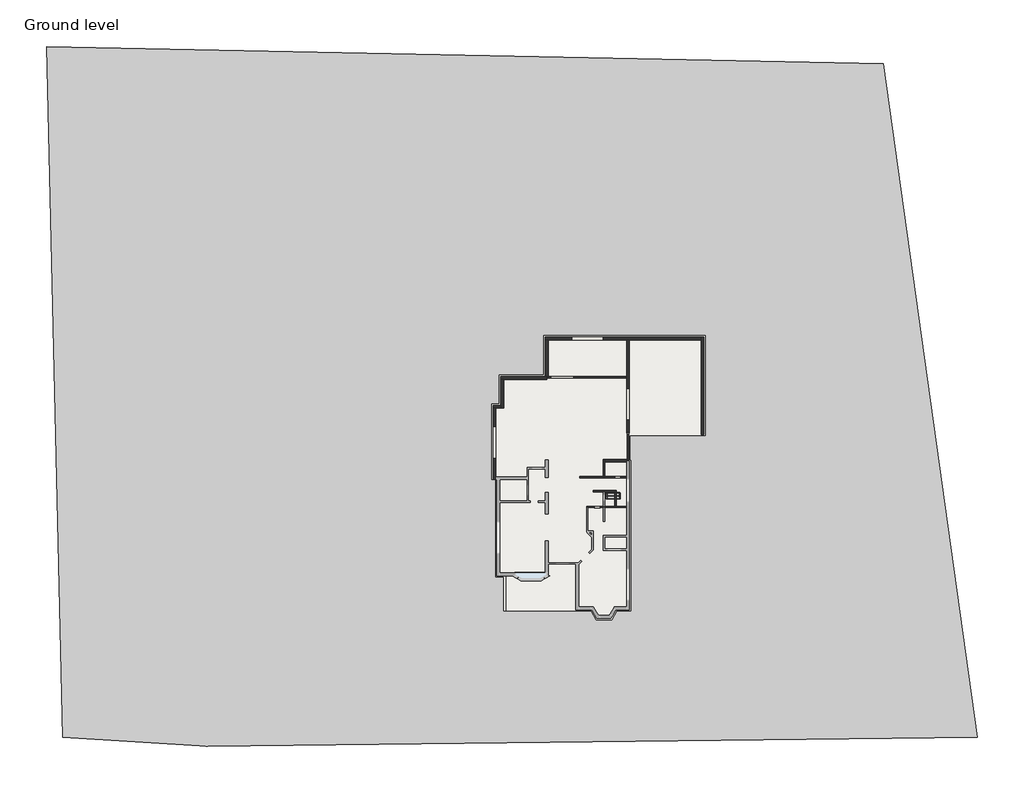
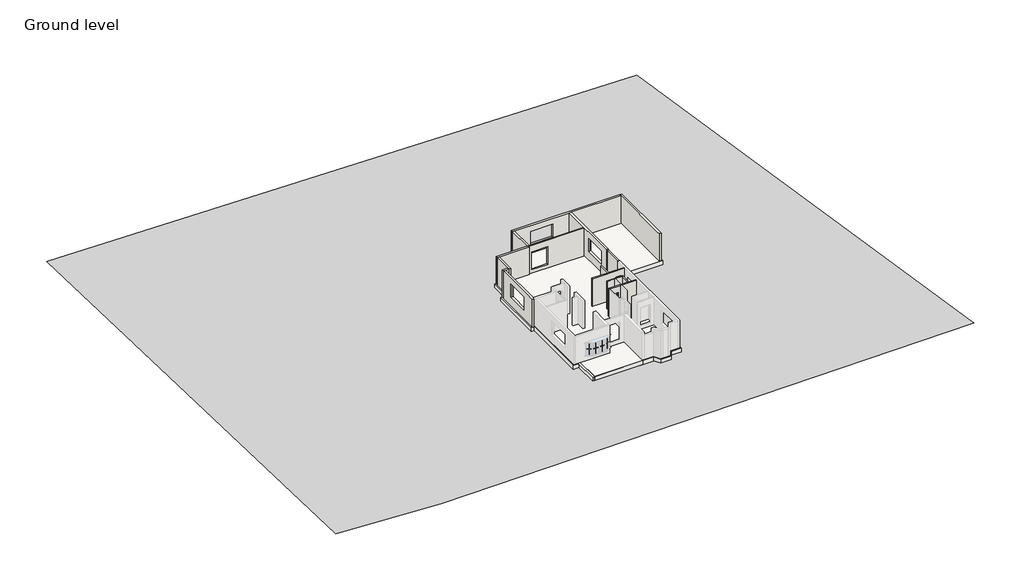
# One storey, part 2 of 2: 16 walls, 6 proxies, 2 members, 2 railings, 2 slabs, 1 stair flight.
"""IFC4 building model written with IfcOpenShell, lengths in millimetres."""

import ifcopenshell
import ifcopenshell.guid

model = None  # the IFC model being written
_history = None  # IfcOwnerHistory: only IFC2X3 demands one
_inside = {}  # id of a spatial element -> (the spatial element, [elements in it])
_under = {}  # id of a project, library or spatial element -> (it, [spatial elements below it])
_declared = {}  # id of a project -> (the project, [libraries it declares])
_typed = {}  # id of a type object -> (the type object, [elements of that type])
_made_of = {}  # id of a material, layer set ... -> (it, [elements and type objects made of it])


def new_model(schema):
    """Start an empty IFC model of exactly this schema.

    Asked for "IFC4X3", IfcOpenShell would pick the latest addendum, in which some entities
    have other attributes; the version numbers below select the first issue.
    IFC2X3 requires an IfcOwnerHistory on every rooted entity: one is made here for all.
    """
    global model, _history
    if schema == "IFC4X3":
        model = ifcopenshell.file(schema_version=(4, 3, 0, 0))
    else:
        model = ifcopenshell.file(schema=schema)
    _inside.clear()
    _under.clear()
    _declared.clear()
    _typed.clear()
    _made_of.clear()
    _history = None
    if model.schema == "IFC2X3":
        org = make("IfcOrganization", Name="unknown")
        user = make(
            "IfcPersonAndOrganization",
            ThePerson=make("IfcPerson", FamilyName="unknown"),
            TheOrganization=org,
        )
        app = make(
            "IfcApplication",
            ApplicationDeveloper=org,
            Version="unknown",
            ApplicationFullName="unknown",
            ApplicationIdentifier="unknown",
        )
        _history = make(
            "IfcOwnerHistory",
            OwningUser=user,
            OwningApplication=app,
            ChangeAction="ADDED",
            CreationDate=0,
        )
    return model


def make(cls, **values):
    """One entity of the class cls with the attributes given. An attribute that is None is left unset."""
    return model.create_entity(
        cls, **{name: value for name, value in values.items() if value is not None}
    )


def rooted(cls, **values):
    """An entity with a GlobalId (a new one), such as an element, a storey or a relation."""
    return make(cls, GlobalId=ifcopenshell.guid.new(), OwnerHistory=_history, **values)


def si_unit(unit_type, name, prefix=None):
    """IfcSIUnit, for example si_unit("LENGTHUNIT", "METRE", prefix="MILLI")."""
    return make("IfcSIUnit", UnitType=unit_type, Prefix=prefix, Name=name)


def assignment(units):
    """IfcUnitAssignment: the units of a project."""
    return None if units is None else make("IfcUnitAssignment", Units=units)


def point(xyz):
    """IfcCartesianPoint."""
    return None if xyz is None else make("IfcCartesianPoint", Coordinates=xyz)


def direction(xyz):
    """IfcDirection."""
    return None if xyz is None else make("IfcDirection", DirectionRatios=xyz)


def frame(location, z_axis=None, x_axis=None):
    """IfcAxis2Placement3D, a coordinate frame: its origin and axes. An axis left out is left unset."""
    return make(
        "IfcAxis2Placement3D",
        Location=point(location),
        Axis=direction(z_axis),
        RefDirection=direction(x_axis),
    )


def frame_2d(location, x_axis=None):
    """IfcAxis2Placement2D, a coordinate frame in the plane: its origin and x axis."""
    return make(
        "IfcAxis2Placement2D", Location=point(location), RefDirection=direction(x_axis)
    )


def origin():
    """The frame at (0, 0, 0) with its axes left unset."""
    return frame((0.0, 0.0, 0.0))


def origin_with_axes():
    """The frame at (0, 0, 0) with the z axis (0, 0, 1) and the x axis (1, 0, 0) written out."""
    return frame((0.0, 0.0, 0.0), z_axis=(0.0, 0.0, 1.0), x_axis=(1.0, 0.0, 0.0))


def place(relative_to, where):
    """IfcLocalPlacement: puts the frame where relative to a parent placement (None: the world)."""
    return make(
        "IfcLocalPlacement", PlacementRelTo=relative_to, RelativePlacement=where
    )


def context(
    kind, dimensions, precision=None, world=None, true_north=None, identifier=None
):
    """IfcGeometricRepresentationContext, for example the 3D "Model" context."""
    return make(
        "IfcGeometricRepresentationContext",
        ContextIdentifier=identifier,
        ContextType=kind,
        CoordinateSpaceDimension=dimensions,
        Precision=precision,
        WorldCoordinateSystem=world,
        TrueNorth=true_north,
    )


def project(units=None, contexts=None):
    """IfcProject with its units and contexts."""
    return rooted(
        "IfcProject",
        Name="project",
        RepresentationContexts=contexts,
        UnitsInContext=assignment(units),
    )


def spatial(cls, under=None, at=None, **own):
    """A site, building, storey or space (cls), placed at a placement, below another one or the project."""
    s = rooted(cls, ObjectPlacement=at, **own)
    if under is not None:
        _under.setdefault(under.id(), (under, []))[1].append(s)
    return s


def polyline(points):
    """IfcPolyline through the points."""
    return make("IfcPolyline", Points=[point(p) for p in points])


def point_list(points):
    """IfcCartesianPointList2D or 3D."""
    cls = (
        "IfcCartesianPointList2D" if len(points[0]) == 2 else "IfcCartesianPointList3D"
    )
    return make(cls, CoordList=points)


def circle_curve(where, radius):
    """IfcCircle in the frame where."""
    return make("IfcCircle", Position=where, Radius=radius)


def trimmed(basis, trim1, trim2, sense, master):
    """IfcTrimmedCurve: the piece of a basis curve between two trims."""
    return make(
        "IfcTrimmedCurve",
        BasisCurve=basis,
        Trim1=trim1,
        Trim2=trim2,
        SenseAgreement=sense,
        MasterRepresentation=master,
    )


def segment(curve, same_sense, transition):
    """IfcCompositeCurveSegment."""
    return make(
        "IfcCompositeCurveSegment",
        Transition=transition,
        SameSense=same_sense,
        ParentCurve=curve,
    )


def composite_curve(segments, self_intersect=None):
    """IfcCompositeCurve: segments joined end to end."""
    return make("IfcCompositeCurve", Segments=segments, SelfIntersect=self_intersect)


def outline(outer, holes=None, kind="AREA"):
    """IfcArbitraryClosedProfileDef: a profile drawn as a closed curve; with holes, ...WithVoids."""
    if holes is None:
        return make("IfcArbitraryClosedProfileDef", ProfileType=kind, OuterCurve=outer)
    return make(
        "IfcArbitraryProfileDefWithVoids",
        ProfileType=kind,
        OuterCurve=outer,
        InnerCurves=holes,
    )


def extrude(swept, where, along, depth):
    """IfcExtrudedAreaSolid: the profile swept, set in the frame where, extruded along a direction by depth."""
    return make(
        "IfcExtrudedAreaSolid",
        SweptArea=swept,
        Position=where,
        ExtrudedDirection=direction(along),
        Depth=depth,
    )


def faces_of(points, faces, orient=None, outer=None):
    """IfcFace entities. A face is a list of loops; a loop is a list of indices into points, from 0.

    orient and outer hold one flag for each loop. By default every Orientation is true, the
    first loop of a face is its IfcFaceOuterBound and the others are IfcFaceBound.
    """
    made = []
    for i, loops in enumerate(faces):
        bounds = []
        for j, loop in enumerate(loops):
            is_outer = j == 0 if outer is None else outer[i][j]
            bounds.append(
                make(
                    "IfcFaceOuterBound" if is_outer else "IfcFaceBound",
                    Bound=make("IfcPolyLoop", Polygon=[points[k] for k in loop]),
                    Orientation=True if orient is None else orient[i][j],
                )
            )
        made.append(make("IfcFace", Bounds=bounds))
    return made


def faceted_brep(points, faces, orient=None, outer=None, voids=None):
    """IfcFacetedBrep: a solid bounded by flat faces; with voids (closed shells), ...WithVoids."""
    shared = [point(p) for p in points]
    hull = make("IfcClosedShell", CfsFaces=faces_of(shared, faces, orient, outer))
    if voids is None:
        return make("IfcFacetedBrep", Outer=hull)
    return make(
        "IfcFacetedBrepWithVoids",
        Outer=hull,
        Voids=[
            make(cls, CfsFaces=faces_of(shared, fs, o, b)) for cls, fs, o, b in voids
        ],
    )


def triangles(points, corners, closed=None, point_numbers=None):
    """IfcTriangulatedFaceSet: each triangle names its three corners, points numbered from 1."""
    return make(
        "IfcTriangulatedFaceSet",
        Coordinates=point_list(points),
        Closed=closed,
        CoordIndex=corners,
        PnIndex=point_numbers,
    )


def shape(context_of_items, identifier, shape_type, items):
    """IfcShapeRepresentation: the items that make up one representation, for example the "Body"."""
    return make(
        "IfcShapeRepresentation",
        ContextOfItems=context_of_items,
        RepresentationIdentifier=identifier,
        RepresentationType=shape_type,
        Items=items,
    )


def source(mapping_origin, context_of_items, identifier, shape_type, items):
    """IfcRepresentationMap: a shape defined once, which mapped items show again and again."""
    return make(
        "IfcRepresentationMap",
        MappingOrigin=mapping_origin,
        MappedRepresentation=shape(context_of_items, identifier, shape_type, items),
    )


def transform(
    local_origin,
    x_axis=None,
    y_axis=None,
    z_axis=None,
    scale=None,
    scale2=None,
    scale3=None,
    uniform=True,
):
    """IfcCartesianTransformationOperator3D, or its non-uniform kind. x_axis, y_axis, z_axis: its Axis1, 2, 3."""
    if uniform:
        return make(
            "IfcCartesianTransformationOperator3D",
            Axis1=direction(x_axis),
            Axis2=direction(y_axis),
            LocalOrigin=point(local_origin),
            Scale=scale,
            Axis3=direction(z_axis),
        )
    return make(
        "IfcCartesianTransformationOperator3DnonUniform",
        Axis1=direction(x_axis),
        Axis2=direction(y_axis),
        LocalOrigin=point(local_origin),
        Scale=scale,
        Axis3=direction(z_axis),
        Scale2=scale2,
        Scale3=scale3,
    )


def mapped(mapping_source, mapping_target):
    """IfcMappedItem: shows the shape of a source again, moved by a transform."""
    return make(
        "IfcMappedItem", MappingSource=mapping_source, MappingTarget=mapping_target
    )


def made_of(thing, what):
    """Note that an element or type object is made of a material, layer set ...; save() writes the relation."""
    if what is not None:
        _made_of.setdefault(what.id(), (what, []))[1].append(thing)
    return thing


def element(
    cls,
    number,
    at=None,
    inside=None,
    cuts=None,
    type_object=None,
    material=None,
    context=None,
    identifier="Body",
    shape_type=None,
    held_by="IfcProductDefinitionShape",
    body=None,
    shapes=None,
    **own,
):
    """One element of the class cls, such as IfcWall. Its Tag is "e" and its number.

    at: its placement. inside: the storey or other place that contains it. cuts: it is an
    opening in that element (IfcRelVoidsElement). A single representation is given by context,
    identifier, shape_type and body (its items); several are given by shapes. held_by: the class
    of the entity that holds the representations. save() writes the other relations.
    """
    e = rooted(cls, Tag="e%d" % number, ObjectPlacement=at, **own)
    if body is not None:
        shapes = [shape(context, identifier, shape_type, body)]
    if shapes is not None:
        e.Representation = make(held_by, Representations=shapes)
    if inside is not None:
        _inside.setdefault(inside.id(), (inside, []))[1].append(e)
    if cuts is not None:
        rooted(
            "IfcRelVoidsElement", RelatingBuildingElement=cuts, RelatedOpeningElement=e
        )
    if type_object is not None:
        _typed.setdefault(type_object.id(), (type_object, []))[1].append(e)
    return made_of(e, material)


def aggregate(whole, parts):
    """IfcRelAggregates: a whole, such as a stair, and the parts it consists of."""
    return rooted("IfcRelAggregates", RelatingObject=whole, RelatedObjects=parts)


def save(model, path):
    """Write the relations noted so far, then the file.

    IfcRelAggregates (storeys below a building ...), IfcRelContainedInSpatialStructure (elements
    in a storey), IfcRelDefinesByType, IfcRelAssociatesMaterial and IfcRelDeclares: one each for
    every whole, place, type object, material and project.
    """
    for whole, parts in _under.values():
        aggregate(whole, parts)
    for where, things in _inside.values():
        rooted(
            "IfcRelContainedInSpatialStructure",
            RelatedElements=things,
            RelatingStructure=where,
        )
    for kind, things in _typed.values():
        rooted("IfcRelDefinesByType", RelatedObjects=things, RelatingType=kind)
    for what, things in _made_of.values():
        rooted("IfcRelAssociatesMaterial", RelatedObjects=things, RelatingMaterial=what)
    for by, libraries in _declared.values():
        rooted("IfcRelDeclares", RelatingContext=by, RelatedDefinitions=libraries)
    model.write(path)


def m_muntin_pattern_2x2_m_muntin_pattern_2x2_0b9f2fee(model_context):
    return source(origin(), model_context, "Body", "SweptSolid", [
        extrude(outline(polyline([(686.5, -6.35), (686.5, -246.1999152), (673.8, -246.1999152), (673.8, -6.35), (0.0, -6.35), (0.0, 6.35), (673.8, 6.35), (673.8, 246.1999152), (686.5, 246.1999152), (686.5, 6.35), (1360.3, 6.35), (1360.3, -6.35), (686.5, -6.35)])), frame((0.0, 9.525, 0.0), z_axis=(0.0, 1.0, 0.0), x_axis=(0.0, 0.0, 1.0)), (0.0, 0.0, 1.0), 12.7),
        extrude(outline(polyline([(686.5, -6.35), (686.5, -246.1999152), (673.8, -246.1999152), (673.8, -6.35), (0.0, -6.35), (0.0, 6.35), (673.8, 6.35), (673.8, 246.1999152), (686.5, 246.1999152), (686.5, 6.35), (1360.3, 6.35), (1360.3, -6.35), (686.5, -6.35)])), frame((0.0, -22.225, 0.0), z_axis=(0.0, 1.0, 0.0), x_axis=(0.0, 0.0, 1.0)), (0.0, 0.0, 1.0), 12.7),
    ])


def m_muntin_pattern_2x2_m_muntin_pattern_2x2_98e5798c(model_context):
    return source(origin(), model_context, "Body", "SweptSolid", [
        extrude(outline(polyline([(686.5, -6.35), (686.5, -223.0), (673.8, -223.0), (673.8, -6.35), (0.0, -6.35), (0.0, 6.35), (673.8, 6.35), (673.8, 223.0), (686.5, 223.0), (686.5, 6.35), (1360.3, 6.35), (1360.3, -6.35), (686.5, -6.35)])), frame((0.0, 9.525, 0.0), z_axis=(0.0, 1.0, 0.0), x_axis=(0.0, 0.0, 1.0)), (0.0, 0.0, 1.0), 12.7),
        extrude(outline(polyline([(686.5, -6.35), (686.5, -223.0), (673.8, -223.0), (673.8, -6.35), (0.0, -6.35), (0.0, 6.35), (673.8, 6.35), (673.8, 223.0), (686.5, 223.0), (686.5, 6.35), (1360.3, 6.35), (1360.3, -6.35), (686.5, -6.35)])), frame((0.0, -22.225, 0.0), z_axis=(0.0, 1.0, 0.0), x_axis=(0.0, 0.0, 1.0)), (0.0, 0.0, 1.0), 12.7),
    ])


def m_muntin_pattern_2x2_m_muntin_pattern_2x2_86194ec4(model_context):
    return source(origin(), model_context, "Body", "SweptSolid", [
        extrude(outline(polyline([(686.5, -6.35), (686.5, -223.0), (673.8, -223.0), (673.8, -6.35), (0.0, -6.35), (0.0, 6.35), (673.8, 6.35), (673.8, 223.0), (686.5, 223.0), (686.5, 6.35), (1360.3, 6.35), (1360.3, -6.35), (686.5, -6.35)])), frame((0.0, -22.225, 0.0), z_axis=(0.0, 1.0, 0.0), x_axis=(0.0, 0.0, 1.0)), (0.0, 0.0, 1.0), 12.7),
        extrude(outline(polyline([(686.5, -6.35), (686.5, -223.0), (673.8, -223.0), (673.8, -6.35), (0.0, -6.35), (0.0, 6.35), (673.8, 6.35), (673.8, 223.0), (686.5, 223.0), (686.5, 6.35), (1360.3, 6.35), (1360.3, -6.35), (686.5, -6.35)])), frame((0.0, 9.525, 0.0), z_axis=(0.0, 1.0, 0.0), x_axis=(0.0, 0.0, 1.0)), (0.0, 0.0, 1.0), 12.7),
    ])


def m_trim_window_interior_flat_picture_frame_cdca9661(model_context):
    return source(origin(), model_context, "Body", "SweptSolid", [
        extrude(outline(polyline([(1297.3, 47.3), (1297.3, -1598.1), (-1297.3, -1598.1), (-1297.3, 47.3), (1297.3, 47.3)]), holes=[polyline([(1237.3, -12.7), (-1237.3, -12.7), (-1237.3, -1538.1), (1237.3, -1538.1), (1237.3, -12.7)])]), origin_with_axes(), (0.0, 0.0, 1.0), 30.0),
    ])


def wood_steps_w_50mm_tread_10mm_nosing_13mm_riser_c9f02b3d(model_context):
    return source(origin(), model_context, "Body", "SweptSolid", [
        extrude(outline(composite_curve([segment(polyline([(-3486.8850615, 150.0), (-3236.8850615, 150.0), (-3236.8850615, 100.0), (-3486.8850615, 100.0), (-3486.8850615, 130.0)]), True, "CONTINUOUS"), segment(trimmed(circle_curve(frame_2d((-3486.8850615, 140.0)), 10.0), [point((-3486.8850615, 130.0))], [point((-3486.8850615, 150.0))], False, "CARTESIAN"), True, "CONTINUOUS")], self_intersect=False)), frame((2002.8766391, 0.0, 0.0), z_axis=(1.0, 0.0, 0.0), x_axis=(0.0, 1.0, 0.0)), (0.0, 0.0, 1.0), 1000.0),
        extrude(outline(polyline([(3002.8766391, -3474.3850615), (3002.8766391, -3486.8850615), (2002.8766391, -3486.8850615), (2002.8766391, -3474.3850615), (3002.8766391, -3474.3850615)])), origin_with_axes(), (0.0, 0.0, 1.0), 100.0),
        extrude(outline(polyline([(3002.8766391, -3224.3850615), (3002.8766391, -3236.8850615), (2002.8766391, -3236.8850615), (2002.8766391, -3224.3850615), (3002.8766391, -3224.3850615)])), frame((0.0, 0.0, 100.0), z_axis=(0.0, 0.0, 1.0), x_axis=(1.0, 0.0, 0.0)), (0.0, 0.0, 1.0), 150.0),
        extrude(outline(polyline([(3002.8766391, -2974.3850615), (3002.8766391, -2986.8850615), (2002.8766391, -2986.8850615), (2002.8766391, -2974.3850615), (3002.8766391, -2974.3850615)])), frame((0.0, 0.0, 250.0), z_axis=(0.0, 0.0, 1.0), x_axis=(1.0, 0.0, 0.0)), (0.0, 0.0, 1.0), 150.0),
        extrude(outline(composite_curve([segment(polyline([(-3236.8850615, 300.0), (-2986.8850615, 300.0), (-2986.8850615, 250.0), (-3236.8850615, 250.0), (-3236.8850615, 280.0)]), True, "CONTINUOUS"), segment(trimmed(circle_curve(frame_2d((-3236.8850615, 290.0)), 10.0), [point((-3236.8850615, 280.0))], [point((-3236.8850615, 300.0))], False, "CARTESIAN"), True, "CONTINUOUS")], self_intersect=False)), frame((2002.8766391, 0.0, 0.0), z_axis=(1.0, 0.0, 0.0), x_axis=(0.0, 1.0, 0.0)), (0.0, 0.0, 1.0), 1000.0),
    ])


model = new_model("IFC4")

# Units and contexts
model_context = context("Model", 3, world=origin())
ifc_project = project(units=[si_unit("LENGTHUNIT", "METRE", prefix="MILLI")], contexts=[model_context])

# Site, building, storey
site = spatial("IfcSite", under=ifc_project)
building = spatial("IfcBuilding", under=site)
storey = spatial("IfcBuildingStorey", under=building, Name="Ground level", Elevation=0.0)

# Proxies
placement = place(None, origin())
element("IfcBuildingElementProxy", 1, Name="Building Element Proxy", at=placement, inside=storey, context=model_context, shape_type="Tessellation", body=[
    triangles([(-42378.2132812, 32370.4567017, -506.3607347), (23861.3784119, 30990.4641907, -506.3607347), (31336.3337769, -22369.2090271, -506.3607347), (-29613.2924377, -23059.2041199, -506.3607347), (-40998.2230957, -20759.218927, -506.3607347), (-41113.2207275, -22369.2090271, -506.3607347)], [[1, 6, 5], [5, 6, 4], [1, 5, 4], [4, 3, 2], [4, 2, 1]], closed=False),
])
m_muntin_pattern_2x2_m_muntin_pattern_2x2_shape = m_muntin_pattern_2x2_m_muntin_pattern_2x2_0b9f2fee(model_context)
element("IfcBuildingElementProxy", 2, Name="M_Muntin Pattern_2x2 : M_Muntin Pattern_2x2", ObjectType="M_Muntin Pattern_2x2 : M_Muntin Pattern_2x2", at=placement, inside=storey, context=model_context, shape_type="MappedRepresentation", body=[
    mapped(m_muntin_pattern_2x2_m_muntin_pattern_2x2_shape, transform((-3655.0691772, -9871.8610544, 720.65), x_axis=(-1.0, 0.0, 0.0), y_axis=(0.0, -1.0, 0.0), z_axis=(0.0, 0.0, 1.0))),
])
element("IfcBuildingElementProxy", 3, Name="M_Muntin Pattern_2x2 : M_Muntin Pattern_2x2", ObjectType="M_Muntin Pattern_2x2 : M_Muntin Pattern_2x2", at=placement, inside=storey, context=model_context, shape_type="MappedRepresentation", body=[
    mapped(m_muntin_pattern_2x2_m_muntin_pattern_2x2_shape, transform((-4388.7690077, -9871.8610544, 720.65), x_axis=(-1.0, 0.0, 0.0), y_axis=(0.0, -1.0, 0.0), z_axis=(0.0, 0.0, 1.0))),
])
m_muntin_pattern_2x2_m_muntin_pattern_2x2_2_shape = m_muntin_pattern_2x2_m_muntin_pattern_2x2_98e5798c(model_context)
element("IfcBuildingElementProxy", 4, Name="M_Muntin Pattern_2x2 : M_Muntin Pattern_2x2", ObjectType="M_Muntin Pattern_2x2 : M_Muntin Pattern_2x2", at=placement, inside=storey, context=model_context, shape_type="MappedRepresentation", body=[
    mapped(m_muntin_pattern_2x2_m_muntin_pattern_2x2_2_shape, transform((-2995.3721319, -9701.3121624, 720.65), x_axis=(-0.8660254037844438, -0.4999999999999912, 0.0), y_axis=(0.4999999999999912, -0.8660254037844438, 0.0), z_axis=(0.0, 0.0, 1.0))),
])
m_muntin_pattern_2x2_m_muntin_pattern_2x2_3_shape = m_muntin_pattern_2x2_m_muntin_pattern_2x2_86194ec4(model_context)
element("IfcBuildingElementProxy", 5, Name="M_Muntin Pattern_2x2 : M_Muntin Pattern_2x2", ObjectType="M_Muntin Pattern_2x2 : M_Muntin Pattern_2x2", at=placement, inside=storey, context=model_context, shape_type="MappedRepresentation", body=[
    mapped(m_muntin_pattern_2x2_m_muntin_pattern_2x2_3_shape, transform((-5048.4660529, -9701.3121624, 720.65), x_axis=(0.8660254037844407, -0.4999999999999965, 0.0), y_axis=(0.4999999999999965, 0.8660254037844407, 0.0), z_axis=(0.0, 0.0, 1.0))),
])
m_trim_window_interior_flat_picture_frame_shape = m_trim_window_interior_flat_picture_frame_cdca9661(model_context)
element("IfcBuildingElementProxy", 6, Name="M_Trim-Window-Interior-Flat : Picture Frame", ObjectType="M_Trim-Window-Interior-Flat : Picture Frame", at=placement, inside=storey, context=model_context, shape_type="MappedRepresentation", body=[
    mapped(m_trim_window_interior_flat_picture_frame_shape, transform((-4021.9190924, -9333.1360544, 2150.8), x_axis=(-1.0, 0.0, 0.0), y_axis=(0.0, 0.0, 1.0), z_axis=(0.0, 1.0, 0.0))),
])

# Members
element("IfcMember", 7, ObjectType="Stringer-50mm_Width", at=placement, inside=storey, context=model_context, shape_type="SweptSolid", body=[
    extrude(outline(polyline([(-3496.8850615, 0.0), (-3496.8850615, 225.715214), (-2996.8850615, 525.715214), (-2996.8850615, 59.2390624), (-3095.6168322, 0.0), (-3496.8850615, 0.0)])), frame((1952.8766391, 0.0, 0.0), z_axis=(1.0, 0.0, 0.0), x_axis=(0.0, 1.0, 0.0)), (0.0, 0.0, 1.0), 50.0),
])
element("IfcMember", 8, ObjectType="Stringer-50mm_Width", at=placement, inside=storey, context=model_context, shape_type="SweptSolid", body=[
    extrude(outline(polyline([(-3496.8850615, 0.0), (-3496.8850615, 225.715214), (-2996.8850615, 525.715214), (-2996.8850615, 59.2390624), (-3095.6168322, 0.0), (-3496.8850615, 0.0)])), frame((3002.8766391, 0.0, 0.0), z_axis=(1.0, 0.0, 0.0), x_axis=(0.0, 1.0, 0.0)), (0.0, 0.0, 1.0), 50.0),
])

# Railings
element("IfcRailing", 9, ObjectType="1100mm", at=placement, inside=storey, context=model_context, shape_type="SweptSolid", body=[
    extrude(outline(polyline([(-3496.8850615, 1191.6904811), (-3496.8850615, 1250.0), (-2996.8850615, 1550.0), (-2996.8850615, 1491.6904811), (-3496.8850615, 1191.6904811)])), frame((2952.4766391, 0.0, 0.0), z_axis=(1.0, 0.0, 0.0), x_axis=(0.0, 1.0, 0.0)), (0.0, 0.0, 1.0), 50.0),
    extrude(outline(polyline([(-3071.8850615, 300.0), (-3071.8850615, 1446.6904811), (-3046.8850615, 1461.6904811), (-3046.8850615, 300.0), (-3071.8850615, 300.0)])), frame((2964.9766391, 0.0, 0.0), z_axis=(1.0, 0.0, 0.0), x_axis=(0.0, 1.0, 0.0)), (0.0, 0.0, 1.0), 25.0),
    extrude(outline(polyline([(-3196.8850615, 300.0), (-3196.8850615, 1371.6904811), (-3171.8850615, 1386.6904811), (-3171.8850615, 300.0), (-3196.8850615, 300.0)])), frame((2964.9766391, 0.0, 0.0), z_axis=(1.0, 0.0, 0.0), x_axis=(0.0, 1.0, 0.0)), (0.0, 0.0, 1.0), 25.0),
    extrude(outline(polyline([(-3321.8850615, 150.0), (-3321.8850615, 1296.6904811), (-3296.8850615, 1311.6904811), (-3296.8850615, 150.0), (-3321.8850615, 150.0)])), frame((2964.9766391, 0.0, 0.0), z_axis=(1.0, 0.0, 0.0), x_axis=(0.0, 1.0, 0.0)), (0.0, 0.0, 1.0), 25.0),
    extrude(outline(polyline([(-3446.8850615, 150.0), (-3446.8850615, 1221.6904811), (-3421.8850615, 1236.6904811), (-3421.8850615, 150.0), (-3446.8850615, 150.0)])), frame((2964.9766391, 0.0, 0.0), z_axis=(1.0, 0.0, 0.0), x_axis=(0.0, 1.0, 0.0)), (0.0, 0.0, 1.0), 25.0),
    extrude(outline(polyline([(-3021.8850615, 300.0), (-3021.8850615, 1476.6904811), (-2996.8850615, 1491.6904811), (-2996.8850615, 300.0), (-3021.8850615, 300.0)])), frame((2964.9766391, 0.0, 0.0), z_axis=(1.0, 0.0, 0.0), x_axis=(0.0, 1.0, 0.0)), (0.0, 0.0, 1.0), 25.0),
    extrude(outline(polyline([(-3496.8850615, 150.0), (-3496.8850615, 1191.6904811), (-3471.8850615, 1206.6904811), (-3471.8850615, 150.0), (-3496.8850615, 150.0)])), frame((2964.9766391, 0.0, 0.0), z_axis=(1.0, 0.0, 0.0), x_axis=(0.0, 1.0, 0.0)), (0.0, 0.0, 1.0), 25.0),
])
element("IfcRailing", 10, ObjectType="1100mm", at=placement, inside=storey, context=model_context, shape_type="SweptSolid", body=[
    extrude(outline(polyline([(-3496.8850615, 1191.6904811), (-3496.8850615, 1250.0), (-2996.8850615, 1550.0), (-2996.8850615, 1491.6904811), (-3496.8850615, 1191.6904811)])), frame((2003.2766391, 0.0, 0.0), z_axis=(1.0, 0.0, 0.0), x_axis=(0.0, 1.0, 0.0)), (0.0, 0.0, 1.0), 50.0),
    extrude(outline(polyline([(-3071.8850615, 1446.6904811), (-3046.8850615, 1461.6904811), (-3046.8850615, 300.0), (-3071.8850615, 300.0), (-3071.8850615, 1446.6904811)])), frame((2015.7766391, 0.0, 0.0), z_axis=(1.0, 0.0, 0.0), x_axis=(0.0, 1.0, 0.0)), (0.0, 0.0, 1.0), 25.0),
    extrude(outline(polyline([(-3196.8850615, 1371.6904811), (-3171.8850615, 1386.6904811), (-3171.8850615, 300.0), (-3196.8850615, 300.0), (-3196.8850615, 1371.6904811)])), frame((2015.7766391, 0.0, 0.0), z_axis=(1.0, 0.0, 0.0), x_axis=(0.0, 1.0, 0.0)), (0.0, 0.0, 1.0), 25.0),
    extrude(outline(polyline([(-3321.8850615, 1296.6904811), (-3296.8850615, 1311.6904811), (-3296.8850615, 150.0), (-3321.8850615, 150.0), (-3321.8850615, 1296.6904811)])), frame((2015.7766391, 0.0, 0.0), z_axis=(1.0, 0.0, 0.0), x_axis=(0.0, 1.0, 0.0)), (0.0, 0.0, 1.0), 25.0),
    extrude(outline(polyline([(-3446.8850615, 1221.6904811), (-3421.8850615, 1236.6904811), (-3421.8850615, 150.0), (-3446.8850615, 150.0), (-3446.8850615, 1221.6904811)])), frame((2015.7766391, 0.0, 0.0), z_axis=(1.0, 0.0, 0.0), x_axis=(0.0, 1.0, 0.0)), (0.0, 0.0, 1.0), 25.0),
    extrude(outline(polyline([(-3021.8850615, 1476.6904811), (-2996.8850615, 1491.6904811), (-2996.8850615, 300.0), (-3021.8850615, 300.0), (-3021.8850615, 1476.6904811)])), frame((2015.7766391, 0.0, 0.0), z_axis=(1.0, 0.0, 0.0), x_axis=(0.0, 1.0, 0.0)), (0.0, 0.0, 1.0), 25.0),
    extrude(outline(polyline([(-3496.8850615, 1191.6904811), (-3471.8850615, 1206.6904811), (-3471.8850615, 150.0), (-3496.8850615, 150.0), (-3496.8850615, 1191.6904811)])), frame((2015.7766391, 0.0, 0.0), z_axis=(1.0, 0.0, 0.0), x_axis=(0.0, 1.0, 0.0)), (0.0, 0.0, 1.0), 25.0),
])

# Slabs
element("IfcSlab", 11, ObjectType="Floor-Grnd-Susp_65Scr-80Ins-100Blk-75PC", at=placement, inside=storey, context=model_context, shape_type="SweptSolid", body=[
    extrude(outline(polyline([(9777.0601381, 9456.2639456), (9777.0601381, 1533.2639456), (3820.4309076, 1533.2639456), (3820.4309076, -448.1360544), (3877.9309076, -448.1360544), (3877.9309076, -12347.8360544), (2762.9750493, -12347.8360544), (2373.2636176, -13040.6563774), (1141.7986672, -13040.6563774), (741.7986672, -12347.8360544), (-6186.6190924, -12347.8360544), (-6186.6190924, -9663.1360544), (-6820.0190924, -9663.1360544), (-6820.0190924, -1948.1360544), (-7124.8190924, -1948.1360544), (-7124.8190924, 4046.0639456), (-6515.2190924, 4046.0639456), (-6515.2190924, 6332.0639456), (-2987.0690924, 6332.0639456), (-2987.0690924, 9456.2639456), (9777.0601381, 9456.2639456)])), frame((0.0, 0.0, -450.0), z_axis=(0.0, 0.0, 1.0), x_axis=(1.0, 0.0, 0.0)), (0.0, 0.0, 1.0), 450.0),
])
element("IfcSlab", 12, ObjectType="Floor-Grnd-Susp_65Scr-80Ins-100Blk-75PC", at=placement, inside=storey, context=model_context, shape_type="SweptSolid", body=[
    extrude(outline(polyline([(-5956.6190924, -12347.8360544), (-5956.6190924, -9563.1360544), (-2641.9190924, -9563.1360544), (-2641.9190924, -8640.6860544), (-471.6190924, -8640.6860544), (-471.6190924, -12347.8360544), (-5956.6190924, -12347.8360544)])), frame((0.0, 0.0, -450.0), z_axis=(0.0, 0.0, 1.0), x_axis=(1.0, 0.0, 0.0)), (0.0, 0.0, 1.0), 450.0),
])

# Stair flight
wood_steps_w_50mm_tread_10mm_nosing_13mm_riser_shape = wood_steps_w_50mm_tread_10mm_nosing_13mm_riser_c9f02b3d(model_context)
element("IfcStairFlight", 13, ObjectType="Wood_Steps_w-50mm_Tread-10mm_Nosing-13mm_Riser", at=placement, inside=storey, context=model_context, shape_type="MappedRepresentation", body=[
    mapped(wood_steps_w_50mm_tread_10mm_nosing_13mm_riser_shape, transform((0.0, 0.0, 0.0), x_axis=(1.0, 0.0, 0.0), y_axis=(0.0, 1.0, 0.0), z_axis=(0.0, 0.0, 1.0))),
])

# Walls
element("IfcWall", 14, ObjectType="Wall-Fnd_115m 2", at=placement, inside=storey, context=model_context, shape_type="Brep", body=[
    faceted_brep([(3720.4309076, -450.5860544, 3327.4), (3720.4309076, -450.5860544, 0.0), (3720.4309076, 1748.2639456, 0.0), (3720.4309076, 1748.2639456, 450.0), (3720.4309076, 1633.2639456, 450.0), (3720.4309076, 1633.2639456, 3327.4), (3605.4309076, -450.5860544, 0.0), (3605.4309076, -450.5860544, 1294.5462794), (3605.4309076, -450.5860544, 3327.4), (3605.4309076, 1633.2639456, 3327.4), (3605.4309076, 1633.2639456, 450.0), (3605.4309076, 1748.2639456, 450.0), (3605.4309076, 1748.2639456, 0.0), (3605.4309076, -335.5860544, 0.0)], [[[0, 1, 2, 3, 4, 5]], [[6, 7, 8, 9, 10, 11, 12, 13]], [[2, 1, 6, 13, 12]], [[0, 5, 9, 8]], [[0, 8, 7, 6, 1]], [[3, 2, 12, 11]], [[10, 4, 3, 11]], [[5, 4, 10, 9]]]),
])
element("IfcWall", 15, ObjectType="Wall-Fnd_115m 2", at=placement, inside=storey, context=model_context, shape_type="Brep", body=[
    faceted_brep([(1700.4309076, -335.5860544, 0.0), (1700.4309076, -1693.0860544, 0.0), (1700.4309076, -1693.0860544, 3327.4), (1700.4309076, -335.5860544, 3327.4), (1815.4309076, -335.5860544, 0.0), (1815.4309076, -335.5860544, 1294.5462794), (1815.4309076, -335.5860544, 3327.4), (1815.4309076, -1693.0860544, 3327.4), (1815.4309076, -1693.0860544, 0.0), (1815.4309076, -565.5860544, 0.0)], [[[0, 1, 2, 3]], [[4, 5, 6, 7, 8, 9]], [[1, 0, 4, 9, 8]], [[3, 2, 7, 6]], [[2, 1, 8, 7]], [[0, 3, 6, 5, 4]]]),
])
element("IfcWall", 16, ObjectType="Wall-Fnd_115m 2", at=placement, inside=storey, context=model_context, shape_type="Brep", body=[
    faceted_brep([(-140.7190924, -1808.0860544, 0.0), (3547.9309076, -1808.0860544, 0.0), (3547.9309076, -1808.0860544, 3327.4), (-140.7190924, -1808.0860544, 3327.4), (3091.4809076, -1808.0860544, 450.0), (2611.4809076, -1808.0860544, 450.0), (2611.4809076, -1808.0860544, 2560.0), (3091.4809076, -1808.0860544, 2560.0), (-140.7190924, -1693.0860544, 0.0), (-140.7190924, -1693.0860544, 3327.4), (1700.4309076, -1693.0860544, 3327.4), (1815.4309076, -1693.0860544, 3327.4), (3547.9309076, -1693.0860544, 3327.4), (3547.9309076, -1693.0860544, 0.0), (1815.4309076, -1693.0860544, 0.0), (1700.4309076, -1693.0860544, 0.0), (3091.4809076, -1693.0860544, 450.0), (3091.4809076, -1693.0860544, 2560.0), (2611.4809076, -1693.0860544, 2560.0), (2611.4809076, -1693.0860544, 450.0)], [[[0, 1, 2, 3], [4, 5, 6, 7]], [[8, 9, 10, 11, 12, 13, 14, 15], [16, 17, 18, 19]], [[1, 0, 8, 15, 14, 13]], [[3, 2, 12, 11, 10, 9]], [[0, 3, 9, 8]], [[17, 16, 4, 7]], [[18, 17, 7, 6]], [[19, 18, 6, 5]], [[16, 19, 5, 4]], [[2, 1, 13, 12]]]),
])
element("IfcWall", 17, ObjectType="Wall-Fnd_115m 2", at=placement, inside=storey, context=model_context, shape_type="Brep", body=[
    faceted_brep([(900.6809076, -2938.3860544, 0.0), (1720.4010752, -2938.3860544, 0.0), (1835.4010752, -2938.3860544, 0.0), (2614.8309076, -2938.3860544, 0.0), (2729.8309076, -2938.3860544, 0.0), (2729.8309076, -2938.3860544, 3327.4), (2614.8309076, -2938.3860544, 3327.4), (1835.4010752, -2938.3860544, 3327.4), (1720.4010752, -2938.3860544, 3327.4), (900.6809076, -2938.3860544, 3327.4), (900.6809076, -2823.3860544, 0.0), (900.6809076, -2823.3860544, 3327.4), (2729.8309076, -2823.3860544, 3327.4), (2729.8309076, -2823.3860544, 0.0)], [[[0, 1, 2, 3, 4, 5, 6, 7, 8, 9]], [[10, 11, 12, 13]], [[4, 3, 2, 1, 0, 10, 13]], [[9, 8, 7, 6, 5, 12, 11]], [[0, 9, 11, 10]], [[5, 4, 13, 12]]]),
])
element("IfcWall", 18, ObjectType="Wall-Fnd_115m 2", at=placement, inside=storey, context=model_context, shape_type="SweptSolid", body=[
    extrude(outline(polyline([(2614.8309076, -4055.2860544), (2614.8309076, -2938.3860544), (2729.8309076, -2938.3860544), (2729.8309076, -4055.2860544), (2614.8309076, -4055.2860544)])), origin_with_axes(), (0.0, 0.0, 1.0), 3327.4),
])
element("IfcWall", 19, ObjectType="Wall-Fnd_115m 2", at=placement, inside=storey, context=model_context, shape_type="Brep", body=[
    faceted_brep([(3547.9309076, -4055.2860544, 0.0), (2729.8309076, -4055.2860544, 0.0), (2614.8309076, -4055.2860544, 0.0), (1835.4010752, -4055.2860544, 0.0), (1720.4010752, -4055.2860544, 0.0), (378.4041712, -4055.2860544, 0.0), (378.4041712, -4055.2860544, 3327.4), (1720.4010752, -4055.2860544, 3327.4), (1835.4010752, -4055.2860544, 3327.4), (2614.8309076, -4055.2860544, 3327.4), (2729.8309076, -4055.2860544, 3327.4), (3547.9309076, -4055.2860544, 3327.4), (1473.4041712, -4055.2860544, 450.0), (1473.4041712, -4055.2860544, 2560.0), (993.4041712, -4055.2860544, 2560.0), (993.4041712, -4055.2860544, 450.0), (3547.9309076, -4170.2860544, 0.0), (3547.9309076, -4170.2860544, 3327.4), (1835.4010752, -4170.2860544, 3327.4), (1720.4010752, -4170.2860544, 3327.4), (493.4041712, -4170.2860544, 3327.4), (378.4041712, -4170.2860544, 3327.4), (378.4041712, -4170.2860544, 0.0), (493.4041712, -4170.2860544, 0.0), (1720.4010752, -4170.2860544, 0.0), (1835.4010752, -4170.2860544, 0.0), (1473.4041712, -4170.2860544, 450.0), (993.4041712, -4170.2860544, 450.0), (993.4041712, -4170.2860544, 2560.0), (1473.4041712, -4170.2860544, 2560.0)], [[[0, 1, 2, 3, 4, 5, 6, 7, 8, 9, 10, 11], [12, 13, 14, 15]], [[16, 17, 18, 19, 20, 21, 22, 23, 24, 25], [26, 27, 28, 29]], [[5, 4, 3, 2, 1, 0, 16, 25, 24, 23, 22]], [[11, 10, 9, 8, 7, 6, 21, 20, 19, 18, 17]], [[6, 5, 22, 21]], [[0, 11, 17, 16]], [[13, 12, 26, 29]], [[14, 13, 29, 28]], [[15, 14, 28, 27]], [[12, 15, 27, 26]]]),
])
element("IfcWall", 20, ObjectType="Wall-Fnd_115m 2", at=placement, inside=storey, context=model_context, shape_type="Brep", body=[
    faceted_brep([(3487.9309076, 6219.0139456, 0.0), (-2657.0690924, 6219.0139456, 0.0), (-2772.0690924, 6219.0139456, 0.0), (-2772.0690924, 6219.0139456, 3327.4), (-2657.0690924, 6219.0139456, 3327.4), (3487.9309076, 6219.0139456, 3327.4), (-2457.0690924, 6219.0139456, 2560.0), (-2457.0690924, 6219.0139456, 450.0), (-647.0690924, 6219.0139456, 450.0), (-647.0690924, 6219.0139456, 2560.0), (3487.9309076, 6104.0139456, 0.0), (3487.9309076, 6104.0139456, 3327.4), (-2772.0690924, 6104.0139456, 3327.4), (-2772.0690924, 6104.0139456, 0.0), (-2457.0690924, 6104.0139456, 2560.0), (-647.0690924, 6104.0139456, 2560.0), (-647.0690924, 6104.0139456, 450.0), (-2457.0690924, 6104.0139456, 450.0)], [[[0, 1, 2, 3, 4, 5], [6, 7, 8, 9]], [[10, 11, 12, 13], [14, 15, 16, 17]], [[2, 1, 0, 10, 13]], [[3, 2, 13, 12]], [[5, 4, 3, 12, 11]], [[0, 5, 11, 10]], [[7, 6, 14, 17]], [[8, 7, 17, 16]], [[9, 8, 16, 15]], [[6, 9, 15, 14]]]),
])
element("IfcWall", 21, ObjectType="Wall-Fnd_230mm 2", at=placement, inside=storey, context=model_context, shape_type="Brep", body=[
    faceted_brep([(-6415.2190924, 6002.0639456, 0.0), (-6185.2190924, 6002.0639456, 0.0), (-2772.0690924, 6002.0639456, 0.0), (-2772.0690924, 6002.0639456, 3327.4), (-6185.2190924, 6002.0639456, 3327.4), (-6415.2190924, 6002.0639456, 3327.4), (-6415.2190924, 6232.0639456, 0.0), (-6415.2190924, 6232.0639456, 3327.4), (-2887.0690924, 6232.0639456, 3327.4), (-2772.0690924, 6232.0639456, 3327.4), (-2772.0690924, 6232.0639456, 0.0), (-2887.0690924, 6232.0639456, 0.0), (-2772.0690924, 6219.0139456, 0.0), (-2772.0690924, 6104.0139456, 0.0), (-2772.0690924, 6219.0139456, 3327.4), (-2772.0690924, 6104.0139456, 3327.4)], [[[0, 1, 2, 3, 4, 5]], [[6, 7, 8, 9, 10, 11]], [[2, 1, 0, 6, 11, 10, 12, 13]], [[3, 2, 13, 12, 10, 9, 14, 15]], [[5, 4, 3, 15, 14, 9, 8, 7]], [[0, 5, 7, 6]]]),
])
element("IfcWall", 22, ObjectType="Wall-Fnd_230mm 2", at=placement, inside=storey, context=model_context, shape_type="Brep", body=[
    faceted_brep([(-2887.0690924, 9126.2639456, 0.0), (-2657.0690924, 9126.2639456, 0.0), (3547.9309076, 9126.2639456, 0.0), (3777.9309076, 9126.2639456, 0.0), (9447.0601381, 9126.2639456, 0.0), (9447.0601381, 9126.2639456, 3327.4), (3777.9309076, 9126.2639456, 3327.4), (3547.9309076, 9126.2639456, 3327.4), (-2657.0690924, 9126.2639456, 3327.4), (-2887.0690924, 9126.2639456, 3327.4), (-804.5690924, 9126.2639456, 2600.8), (1695.4309076, 9126.2639456, 2600.8), (1695.4309076, 9126.2639456, 1050.0), (-804.5690924, 9126.2639456, 1050.0), (-2887.0690924, 9356.2639456, 0.0), (-2887.0690924, 9356.2639456, 3327.4), (9447.0601381, 9356.2639456, 3327.4), (9447.0601381, 9356.2639456, 0.0), (1730.3559076, 9356.2639456, 2600.8), (-839.4940924, 9356.2639456, 2600.8), (-839.4940924, 9356.2639456, 1050.0), (1730.3559076, 9356.2639456, 1050.0), (-804.5690924, 9295.7720712, 2600.8), (1695.4309076, 9295.7720712, 2600.8), (-804.5690924, 9295.7720712, 1050.0), (1695.4309076, 9295.7720712, 1050.0)], [[[0, 1, 2, 3, 4, 5, 6, 7, 8, 9], [10, 11, 12, 13]], [[14, 15, 16, 17], [18, 19, 20, 21]], [[4, 3, 2, 1, 0, 14, 17]], [[9, 8, 7, 6, 5, 16, 15]], [[5, 4, 17, 16]], [[0, 9, 15, 14]], [[22, 19, 18, 23, 11, 10]], [[24, 13, 12, 25, 21, 20]], [[22, 10, 13, 24]], [[11, 23, 25, 12]], [[23, 18, 21, 25]], [[19, 22, 24, 20]]]),
])
element("IfcWall", 23, ObjectType="Wall-Fnd_230mm 2", at=placement, inside=storey, context=model_context, shape_type="Brep", body=[
    faceted_brep([(3547.9309076, 9126.2639456, 0.0), (3547.9309076, 1748.2639456, 0.0), (3547.9309076, 1748.2639456, 450.0), (3547.9309076, 1863.2639456, 450.0), (3547.9309076, 1863.2639456, 3327.4), (3547.9309076, 9126.2639456, 3327.4), (3547.9309076, 5263.2639456, 2600.8), (3547.9309076, 2763.2639456, 2600.8), (3547.9309076, 2763.2639456, 1050.0), (3547.9309076, 5263.2639456, 1050.0), (3777.9309076, 9126.2639456, 0.0), (3777.9309076, 9126.2639456, 3327.4), (3777.9309076, 1863.2639456, 3327.4), (3777.9309076, 1863.2639456, 450.0), (3777.9309076, 1748.2639456, 450.0), (3777.9309076, 1748.2639456, 0.0), (3777.9309076, 2728.3389456, 2600.8), (3777.9309076, 5298.1889456, 2600.8), (3777.9309076, 5298.1889456, 1050.0), (3777.9309076, 2728.3389456, 1050.0), (3720.4309076, 1748.2639456, 0.0), (3605.4309076, 1748.2639456, 0.0), (3720.4309076, 1748.2639456, 450.0), (3605.4309076, 1748.2639456, 450.0), (3717.4390331, 5263.2639456, 2600.8), (3717.4390331, 2763.2639456, 2600.8), (3717.4390331, 5263.2639456, 1050.0), (3717.4390331, 2763.2639456, 1050.0)], [[[0, 1, 2, 3, 4, 5], [6, 7, 8, 9]], [[10, 11, 12, 13, 14, 15], [16, 17, 18, 19]], [[1, 0, 10, 15, 20, 21]], [[5, 4, 12, 11]], [[0, 5, 11, 10]], [[2, 1, 21, 20, 15, 14, 22, 23]], [[13, 3, 2, 23, 22, 14]], [[4, 3, 13, 12]], [[24, 17, 16, 25, 7, 6]], [[26, 9, 8, 27, 19, 18]], [[24, 6, 9, 26]], [[7, 25, 27, 8]], [[25, 16, 19, 27]], [[17, 24, 26, 18]]]),
])
element("IfcWall", 24, ObjectType="Wall-Fnd_230mm 2", at=placement, inside=storey, context=model_context, shape_type="Brep", body=[
    faceted_brep([(9677.0601381, 1633.2639456, 0.0), (9677.0601381, 9356.2639456, 0.0), (9677.0601381, 9356.2639456, 3327.4), (9677.0601381, 1633.2639456, 3327.4), (9447.0601381, 1633.2639456, 0.0), (9447.0601381, 1633.2639456, 450.0), (9447.0601381, 1633.2639456, 3327.4), (9447.0601381, 1863.2639456, 3327.4), (9447.0601381, 9126.2639456, 3327.4), (9447.0601381, 9356.2639456, 3327.4), (9447.0601381, 9356.2639456, 0.0), (9447.0601381, 9126.2639456, 0.0)], [[[0, 1, 2, 3]], [[4, 5, 6, 7, 8, 9, 10, 11]], [[1, 0, 4, 11, 10]], [[3, 2, 9, 8, 7, 6]], [[2, 1, 10, 9]], [[0, 3, 6, 5, 4]]]),
])
element("IfcWall", 25, ObjectType="Wall-Fnd_230mm 2", at=placement, inside=storey, context=model_context, shape_type="Brep", body=[
    faceted_brep([(-6415.2190924, 6002.0639456, 0.0), (-6415.2190924, 3946.0639456, 0.0), (-6415.2190924, 3716.0639456, 0.0), (-6415.2190924, 3716.0639456, 3327.4), (-6415.2190924, 3946.0639456, 3327.4), (-6415.2190924, 6002.0639456, 3327.4), (-6185.2190924, 6002.0639456, 0.0), (-6185.2190924, 6002.0639456, 3327.4), (-6185.2190924, 3716.0639456, 3327.4), (-6185.2190924, 3716.0639456, 0.0)], [[[0, 1, 2, 3, 4, 5]], [[6, 7, 8, 9]], [[2, 1, 0, 6, 9]], [[5, 4, 3, 8, 7]], [[0, 5, 7, 6]], [[3, 2, 9, 8]]]),
])
element("IfcWall", 26, ObjectType="Wall-Fnd_230mm 2", at=placement, inside=storey, context=model_context, shape_type="Brep", body=[
    faceted_brep([(-6415.2190924, 3946.0639456, 0.0), (-7024.8190924, 3946.0639456, 0.0), (-7024.8190924, 3946.0639456, 3327.4), (-6415.2190924, 3946.0639456, 3327.4), (-6415.2190924, 3716.0639456, 0.0), (-6415.2190924, 3716.0639456, 3327.4), (-6794.8190924, 3716.0639456, 3327.4), (-7024.8190924, 3716.0639456, 3327.4), (-7024.8190924, 3716.0639456, 0.0), (-6794.8190924, 3716.0639456, 0.0)], [[[0, 1, 2, 3]], [[4, 5, 6, 7, 8, 9]], [[1, 0, 4, 9, 8]], [[3, 2, 7, 6, 5]], [[0, 3, 5, 4]], [[2, 1, 8, 7]]]),
])
element("IfcWall", 27, ObjectType="Wall-Fnd_230mm 2", at=placement, inside=storey, context=model_context, shape_type="Brep", body=[
    faceted_brep([(-7024.8190924, 3716.0639456, 0.0), (-7024.8190924, -1948.1360544, 0.0), (-7024.8190924, -1948.1360544, 3327.4), (-7024.8190924, 3716.0639456, 3327.4), (-7024.8190924, 2283.8889456, 2600.8), (-7024.8190924, -285.9610544, 2600.8), (-7024.8190924, -285.9610544, 1050.0), (-7024.8190924, 2283.8889456, 1050.0), (-6794.8190924, 3716.0639456, 0.0), (-6794.8190924, 3716.0639456, 3327.4), (-6794.8190924, -1718.1360544, 3327.4), (-6794.8190924, -1948.1360544, 3327.4), (-6794.8190924, -1948.1360544, 0.0), (-6794.8190924, -1718.1360544, 0.0), (-6794.8190924, -251.0360544, 2600.8), (-6794.8190924, 2248.9639456, 2600.8), (-6794.8190924, 2248.9639456, 1050.0), (-6794.8190924, -251.0360544, 1050.0), (-6964.327218, -251.0360544, 2600.8), (-6964.327218, 2248.9639456, 2600.8), (-6964.327218, -251.0360544, 1050.0), (-6964.327218, 2248.9639456, 1050.0)], [[[0, 1, 2, 3], [4, 5, 6, 7]], [[8, 9, 10, 11, 12, 13], [14, 15, 16, 17]], [[1, 0, 8, 13, 12]], [[3, 2, 11, 10, 9]], [[0, 3, 9, 8]], [[2, 1, 12, 11]], [[18, 5, 4, 19, 15, 14]], [[20, 17, 16, 21, 7, 6]], [[18, 14, 17, 20]], [[15, 19, 21, 16]], [[19, 4, 7, 21]], [[5, 18, 20, 6]]]),
])
element("IfcWall", 28, ObjectType="Wall-Fnd_230mm 2", at=placement, inside=storey, context=model_context, shape_type="SweptSolid", body=[
    extrude(outline(polyline([(-2657.0690924, 9126.2639456), (-2657.0690924, 6219.0139456), (-2772.0690924, 6219.0139456), (-2772.0690924, 6232.0639456), (-2887.0690924, 6232.0639456), (-2887.0690924, 9126.2639456), (-2657.0690924, 9126.2639456)])), origin_with_axes(), (0.0, 0.0, 1.0), 3327.4),
])
element("IfcWall", 29, ObjectType="Wall-Fnd_230mm 2", at=placement, inside=storey, context=model_context, shape_type="SweptSolid", body=[
    extrude(outline(polyline([(3547.9309076, -565.5860544), (1815.4309076, -565.5860544), (1815.4309076, -335.5860544), (3605.4309076, -335.5860544), (3605.4309076, -450.5860544), (3547.9309076, -450.5860544), (3547.9309076, -565.5860544)])), origin_with_axes(), (0.0, 0.0, 1.0), 1294.5462794),
])

save(model, "model.ifc")

# Revit data of these elements
# Type "M_Muntin Pattern_2x2 : M_Muntin Pattern_2x2"
#   Width [instance default] = 1200 mm
#   Thickness = 12.7 mm
#   Height [instance default] = 1200 mm
#   Distance = 19.05 mm
#   Interior Material [instance default] = none
#   Exterior Material [instance default] = none
#   Default Elevation = 0
# Type "M_Trim-Window-Interior-Flat : Picture Frame"
#   Trim Thickness_Picture Frame = 30 mm
#   Trim Width = 60 mm
#   Trim Thickness_with Sill = 20 mm
#   Sill Thickness = 30 mm
#   Opening Width [instance default] = 600 mm
#   Opening Height [instance default] = 900 mm
#   Default Elevation = 1200 mm
#   Sill = no
#   Picture Frame = yes
#   Trim Material [instance default] = none
# Type "1100mm"
#   built-in parameter 1008612 = 0.019685 (stored number, unit not read)
#   built-in parameter 1008611 = 0.019685 (stored number, unit not read)
#   built-in parameter 1008609 = 0.902231 (stored number, unit not read)
#   built-in parameter 1008604 = 0.19685 (stored number, unit not read)
#   built-in parameter 1008603 = 0.164042 (stored number, unit not read)
#   Railing Height = 1100 mm
#   built-in parameter 1008630 = 2
#   built-in parameter 1008610 = 2
#   built-in parameter 1008608 = 1
#   built-in parameter 1008618 = Baluster_Square : 25mm
# Type "Floor-Grnd-Susp_65Scr-80Ins-100Blk-75PC"
#   Keynote = "E60/130"
#   Function = 0
#   Layers, outside or top first: 65 mm "Concrete, Sand/Cement Screed" (function 4); 0 mm "Vapor Retarder" (function 100); 80 mm "Rigid insulation" (function 3); 130 mm "Air" (function 3); 0 mm "Damp-proofing" (function 100); 100 mm "Concrete Masonry, Floor Block" (function 1); 75 mm "Concrete, Precast" (function 1)
# Type "Wall-Fnd_115m 2"
#   Keynote = "F10"
#   Layers, outside or top first: 115 mm "Concrete Masonry Units" (function 1)
# Type "Wall-Fnd_230mm 2"
#   Keynote = "F10"
#   Layers, outside or top first: 230 mm "Concrete Masonry Units" (function 1)
# Element 1 (IfcBuildingElementProxy)
#   Material = Concrete, Precast
#   Phase Created = New Construction
# Elements 2, 3 (IfcBuildingElementProxy, "M_Muntin Pattern_2x2 : M_Muntin Pattern_2x2")
#   Width = 492.4 mm
#   Height = 1360.3 mm
#   Interior Material = Wood - Stained
#   Exterior Material = Clad - White
#   Phase Created = New Construction
#   Materials on its faces: "Clad - White", "Wood - Stained"
# Elements 4, 5 (IfcBuildingElementProxy, "M_Muntin Pattern_2x2 : M_Muntin Pattern_2x2")
#   Width = 446 mm
#   Height = 1360.3 mm
#   Interior Material = Wood - Stained
#   Exterior Material = Clad - White
#   Phase Created = New Construction
#   Materials on its faces: "Clad - White", "Wood - Stained"
# Element 6 (IfcBuildingElementProxy, "M_Trim-Window-Interior-Flat : Picture Frame")
#   Opening Width = 2500 mm
#   Opening Height = 1550.8 mm
#   Trim Material = Wood - Stained
#   Phase Created = New Construction
#   Materials on its faces: "Wood - Stained"
# Elements 7, 8 (IfcMember, "Stringer-50mm_Width")
#   Phase Created = New Construction
# Elements 9, 10 (IfcRailing, "1100mm")
#   Phase Created = New Construction
# Element 11 (IfcSlab, "Floor-Grnd-Susp_65Scr-80Ins-100Blk-75PC")
#   Height Offset From Level = 0 mm
#   Phase Created = New Construction
#   Materials on its faces: "Concrete, Precast", "Concrete, Sand/Cement Screed"
# Element 12 (IfcSlab, "Floor-Grnd-Susp_65Scr-80Ins-100Blk-75PC")
#   built-in parameter 1001955 = -1.5708 (stored number, unit not read)
#   Height Offset From Level = 0 mm
#   Phase Created = New Construction
#   Materials on its faces: "Concrete, Precast", "Concrete, Sand/Cement Screed"
# Element 13 (IfcStairFlight, "Wood_Steps_w-50mm_Tread-10mm_Nosing-13mm_Riser")
#   Phase Created = New Construction
#   Materials on its faces: "Oak Flooring"
# Elements 14, 15, 16, 17, 18, 19, 20 (IfcWall, "Wall-Fnd_115m 2")
#   Top Offset = 0 mm
#   Base Offset = 0 mm
#   Unconnected Height = 3327.4 mm
#   wall height = 3327.4 mm
#   Phase Created = New Construction
#   Base Constraint = Ground level
#   Materials on its faces: "Concrete Masonry Units"
# Elements 21, 22, 23, 24, 25, 26, 27, 28 (IfcWall, "Wall-Fnd_230mm 2")
#   Top Offset = 0 mm
#   Base Offset = 0 mm
#   Unconnected Height = 3327.4 mm
#   wall height = 3327.4 mm
#   Phase Created = New Construction
#   Base Constraint = Ground level
#   Materials on its faces: "Concrete Masonry Units"
# Element 29 (IfcWall, "Wall-Fnd_230mm 2")
#   Top Offset = 0 mm
#   Base Offset = 0 mm
#   Unconnected Height = 1294.546 mm
#   wall height = 1294.546 mm
#   Phase Created = New Construction
#   Base Constraint = Ground level
#   Materials on its faces: "Concrete Masonry Units"
# Materials
#   "Concrete, Sand/Cement Screed": class "Concrete", colour RGB 127 127 127, transparency 0, Description = "Concrete slab topping", Cost = 0
#   "Vapor Retarder": class "Generic", colour RGB 120 120 120, transparency 0, Description = "Polyethylene film membrane", Cost = 0
#   "Rigid insulation": class "Generic", colour RGB 127 127 127, transparency 0, Description = "Rigid foam insulation board", Cost = 0
#   "Air": class "Gas", colour RGB 255 255 255, transparency 0, Description = "Air", Cost = 0
#   "Damp-proofing": class "Generic", colour RGB 127 127 127, transparency 0, Description = "Damp-proofing", Cost = 0
#   "Concrete Masonry, Floor Block": class "Concrete", colour RGB 181 181 181, transparency 0, Description = "physical material", Cost = 0
#   "Concrete, Precast": class "Concrete", colour RGB 192 192 192, transparency 0, Description = "Precast concrete", Cost = 0
#   "Concrete Masonry Units": class "Masonry", colour RGB 181 181 181, transparency 0, Description = "Concrete masonry units", Cost = 0
#   "Clad - White": class "Wood", colour RGB 242 242 238, transparency 0, Cost = 0
#   "Wood - Stained": class "Wood", colour RGB 227 170 128, transparency 0, Cost = 0
#   "Oak Flooring": class "Wood", colour RGB 212 179 113, transparency 0, Description = "Quercus Rubra", Cost = 0
